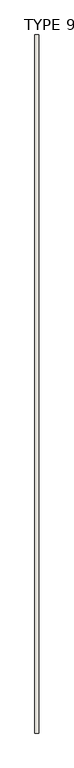
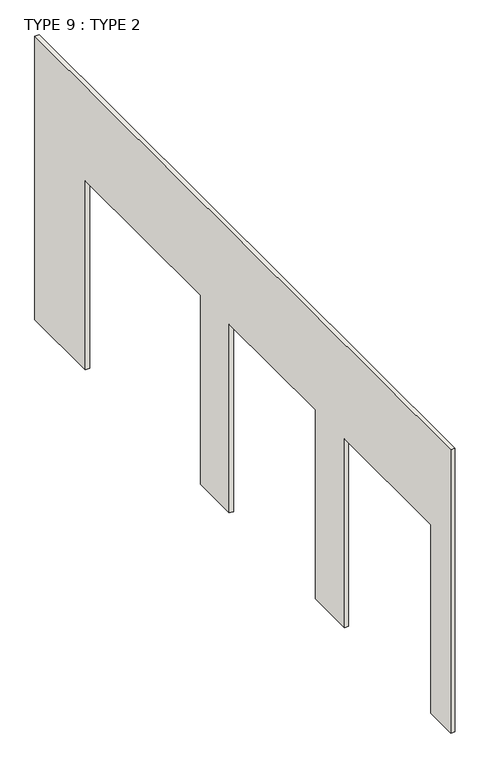
"""IFC4 building model written with IfcOpenShell, lengths in millimetres: wall geometry, TYPE 9 : TYPE 2."""

from ifc_helpers import new_model, si_unit, frame, origin, place, context, project, spatial, polyline, outline, extrude, source, transform, mapped, element, save


def type_9_type_2_6e47f193(model_context):
    return source(origin(), model_context, "Body", "SweptSolid", [
        extrude(outline(polyline([(5418.1649881, 3657.6), (14218.440365, 3657.6), (14218.440365, 0.0), (13151.640365, 0.0), (13151.640365, 2438.4), (10713.240365, 2438.4), (10713.240365, 0.0), (10103.640365, 0.0), (10103.640365, 2438.4), (8274.840365, 2438.4), (8274.840365, 0.0), (7665.240365, 0.0), (7665.240365, 2438.4), (5836.440365, 2438.4), (5836.440365, 0.0), (5418.1649881, 0.0), (5418.1649881, 3657.6)])), frame((-49734.7440345, 0.0, 0.0), z_axis=(1.0, 0.0, 0.0), x_axis=(0.0, 1.0, 0.0)), (0.0, 0.0, 1.0), 50.8),
    ])


if __name__ == "__main__":
    model = new_model("IFC4")
    model_context = context("Model", 3, world=origin())
    ifc_project = project(units=[si_unit("LENGTHUNIT", "METRE", prefix="MILLI")], contexts=[model_context])
    site = spatial("IfcSite", under=ifc_project)
    building = spatial("IfcBuilding", under=site)
    placement = place(None, origin())
    type_9_type_2_shape = type_9_type_2_6e47f193(model_context)
    element("IfcWall", 1, ObjectType="TYPE 9 : TYPE 2", at=placement, inside=building, context=model_context, shape_type="MappedRepresentation", body=[
        mapped(type_9_type_2_shape, transform((0.0, 0.0, 0.0), x_axis=(1.0, 0.0, 0.0), y_axis=(0.0, 1.0, 0.0), z_axis=(0.0, 0.0, 1.0))),
    ])
    save(model, "model.ifc")

# Revit data of these elements
# Element 1 (IfcWall, "TYPE 9 : TYPE 2")
#   Materials on its faces: "Metal"
# Materials
#   "Metal": class "Metal", colour RGB 189 187 185, transparency 0
